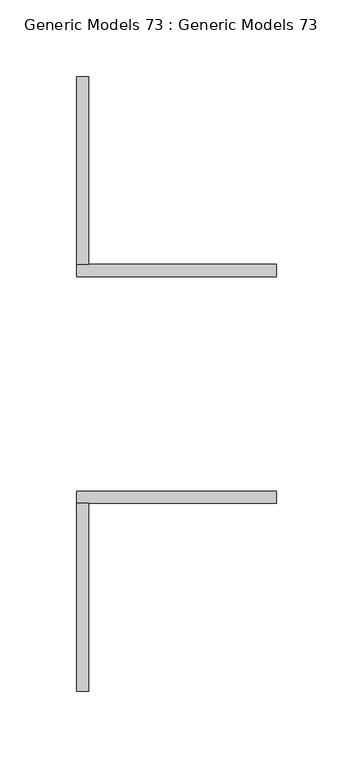
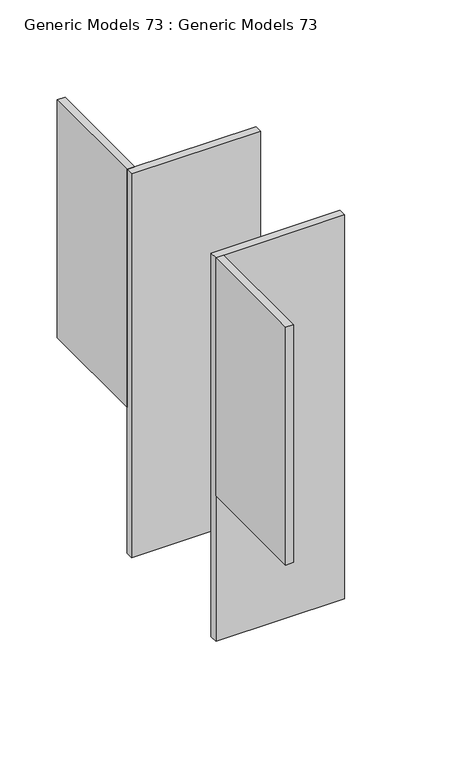
"""IFC4 building model written with IfcOpenShell, lengths in millimetres: proxy geometry, Generic Models 73 : Generic Models 73."""

import ifcopenshell
import ifcopenshell.guid

model = None  # the IFC model being written
_history = None  # IfcOwnerHistory: only IFC2X3 demands one
_inside = {}  # id of a spatial element -> (the spatial element, [elements in it])
_under = {}  # id of a project, library or spatial element -> (it, [spatial elements below it])
_declared = {}  # id of a project -> (the project, [libraries it declares])
_typed = {}  # id of a type object -> (the type object, [elements of that type])
_made_of = {}  # id of a material, layer set ... -> (it, [elements and type objects made of it])


def new_model(schema):
    """Start an empty IFC model of exactly this schema.

    Asked for "IFC4X3", IfcOpenShell would pick the latest addendum, in which some entities
    have other attributes; the version numbers below select the first issue.
    IFC2X3 requires an IfcOwnerHistory on every rooted entity: one is made here for all.
    """
    global model, _history
    if schema == "IFC4X3":
        model = ifcopenshell.file(schema_version=(4, 3, 0, 0))
    else:
        model = ifcopenshell.file(schema=schema)
    _inside.clear()
    _under.clear()
    _declared.clear()
    _typed.clear()
    _made_of.clear()
    _history = None
    if model.schema == "IFC2X3":
        org = make("IfcOrganization", Name="unknown")
        user = make(
            "IfcPersonAndOrganization",
            ThePerson=make("IfcPerson", FamilyName="unknown"),
            TheOrganization=org,
        )
        app = make(
            "IfcApplication",
            ApplicationDeveloper=org,
            Version="unknown",
            ApplicationFullName="unknown",
            ApplicationIdentifier="unknown",
        )
        _history = make(
            "IfcOwnerHistory",
            OwningUser=user,
            OwningApplication=app,
            ChangeAction="ADDED",
            CreationDate=0,
        )
    return model


def make(cls, **values):
    """One entity of the class cls with the attributes given. An attribute that is None is left unset."""
    return model.create_entity(
        cls, **{name: value for name, value in values.items() if value is not None}
    )


def rooted(cls, **values):
    """An entity with a GlobalId (a new one), such as an element, a storey or a relation."""
    return make(cls, GlobalId=ifcopenshell.guid.new(), OwnerHistory=_history, **values)


def si_unit(unit_type, name, prefix=None):
    """IfcSIUnit, for example si_unit("LENGTHUNIT", "METRE", prefix="MILLI")."""
    return make("IfcSIUnit", UnitType=unit_type, Prefix=prefix, Name=name)


def assignment(units):
    """IfcUnitAssignment: the units of a project."""
    return None if units is None else make("IfcUnitAssignment", Units=units)


def point(xyz):
    """IfcCartesianPoint."""
    return None if xyz is None else make("IfcCartesianPoint", Coordinates=xyz)


def direction(xyz):
    """IfcDirection."""
    return None if xyz is None else make("IfcDirection", DirectionRatios=xyz)


def frame(location, z_axis=None, x_axis=None):
    """IfcAxis2Placement3D, a coordinate frame: its origin and axes. An axis left out is left unset."""
    return make(
        "IfcAxis2Placement3D",
        Location=point(location),
        Axis=direction(z_axis),
        RefDirection=direction(x_axis),
    )


def origin():
    """The frame at (0, 0, 0) with its axes left unset."""
    return frame((0.0, 0.0, 0.0))


def place(relative_to, where):
    """IfcLocalPlacement: puts the frame where relative to a parent placement (None: the world)."""
    return make(
        "IfcLocalPlacement", PlacementRelTo=relative_to, RelativePlacement=where
    )


def context(
    kind, dimensions, precision=None, world=None, true_north=None, identifier=None
):
    """IfcGeometricRepresentationContext, for example the 3D "Model" context."""
    return make(
        "IfcGeometricRepresentationContext",
        ContextIdentifier=identifier,
        ContextType=kind,
        CoordinateSpaceDimension=dimensions,
        Precision=precision,
        WorldCoordinateSystem=world,
        TrueNorth=true_north,
    )


def project(units=None, contexts=None):
    """IfcProject with its units and contexts."""
    return rooted(
        "IfcProject",
        Name="project",
        RepresentationContexts=contexts,
        UnitsInContext=assignment(units),
    )


def spatial(cls, under=None, at=None, **own):
    """A site, building, storey or space (cls), placed at a placement, below another one or the project."""
    s = rooted(cls, ObjectPlacement=at, **own)
    if under is not None:
        _under.setdefault(under.id(), (under, []))[1].append(s)
    return s


def polyline(points):
    """IfcPolyline through the points."""
    return make("IfcPolyline", Points=[point(p) for p in points])


def outline(outer, holes=None, kind="AREA"):
    """IfcArbitraryClosedProfileDef: a profile drawn as a closed curve; with holes, ...WithVoids."""
    if holes is None:
        return make("IfcArbitraryClosedProfileDef", ProfileType=kind, OuterCurve=outer)
    return make(
        "IfcArbitraryProfileDefWithVoids",
        ProfileType=kind,
        OuterCurve=outer,
        InnerCurves=holes,
    )


def extrude(swept, where, along, depth):
    """IfcExtrudedAreaSolid: the profile swept, set in the frame where, extruded along a direction by depth."""
    return make(
        "IfcExtrudedAreaSolid",
        SweptArea=swept,
        Position=where,
        ExtrudedDirection=direction(along),
        Depth=depth,
    )


def shape(context_of_items, identifier, shape_type, items):
    """IfcShapeRepresentation: the items that make up one representation, for example the "Body"."""
    return make(
        "IfcShapeRepresentation",
        ContextOfItems=context_of_items,
        RepresentationIdentifier=identifier,
        RepresentationType=shape_type,
        Items=items,
    )


def source(mapping_origin, context_of_items, identifier, shape_type, items):
    """IfcRepresentationMap: a shape defined once, which mapped items show again and again."""
    return make(
        "IfcRepresentationMap",
        MappingOrigin=mapping_origin,
        MappedRepresentation=shape(context_of_items, identifier, shape_type, items),
    )


def transform(
    local_origin,
    x_axis=None,
    y_axis=None,
    z_axis=None,
    scale=None,
    scale2=None,
    scale3=None,
    uniform=True,
):
    """IfcCartesianTransformationOperator3D, or its non-uniform kind. x_axis, y_axis, z_axis: its Axis1, 2, 3."""
    if uniform:
        return make(
            "IfcCartesianTransformationOperator3D",
            Axis1=direction(x_axis),
            Axis2=direction(y_axis),
            LocalOrigin=point(local_origin),
            Scale=scale,
            Axis3=direction(z_axis),
        )
    return make(
        "IfcCartesianTransformationOperator3DnonUniform",
        Axis1=direction(x_axis),
        Axis2=direction(y_axis),
        LocalOrigin=point(local_origin),
        Scale=scale,
        Axis3=direction(z_axis),
        Scale2=scale2,
        Scale3=scale3,
    )


def mapped(mapping_source, mapping_target):
    """IfcMappedItem: shows the shape of a source again, moved by a transform."""
    return make(
        "IfcMappedItem", MappingSource=mapping_source, MappingTarget=mapping_target
    )


def made_of(thing, what):
    """Note that an element or type object is made of a material, layer set ...; save() writes the relation."""
    if what is not None:
        _made_of.setdefault(what.id(), (what, []))[1].append(thing)
    return thing


def element(
    cls,
    number,
    at=None,
    inside=None,
    cuts=None,
    type_object=None,
    material=None,
    context=None,
    identifier="Body",
    shape_type=None,
    held_by="IfcProductDefinitionShape",
    body=None,
    shapes=None,
    **own,
):
    """One element of the class cls, such as IfcWall. Its Tag is "e" and its number.

    at: its placement. inside: the storey or other place that contains it. cuts: it is an
    opening in that element (IfcRelVoidsElement). A single representation is given by context,
    identifier, shape_type and body (its items); several are given by shapes. held_by: the class
    of the entity that holds the representations. save() writes the other relations.
    """
    e = rooted(cls, Tag="e%d" % number, ObjectPlacement=at, **own)
    if body is not None:
        shapes = [shape(context, identifier, shape_type, body)]
    if shapes is not None:
        e.Representation = make(held_by, Representations=shapes)
    if inside is not None:
        _inside.setdefault(inside.id(), (inside, []))[1].append(e)
    if cuts is not None:
        rooted(
            "IfcRelVoidsElement", RelatingBuildingElement=cuts, RelatedOpeningElement=e
        )
    if type_object is not None:
        _typed.setdefault(type_object.id(), (type_object, []))[1].append(e)
    return made_of(e, material)


def aggregate(whole, parts):
    """IfcRelAggregates: a whole, such as a stair, and the parts it consists of."""
    return rooted("IfcRelAggregates", RelatingObject=whole, RelatedObjects=parts)


def save(model, path):
    """Write the relations noted so far, then the file.

    IfcRelAggregates (storeys below a building ...), IfcRelContainedInSpatialStructure (elements
    in a storey), IfcRelDefinesByType, IfcRelAssociatesMaterial and IfcRelDeclares: one each for
    every whole, place, type object, material and project.
    """
    for whole, parts in _under.values():
        aggregate(whole, parts)
    for where, things in _inside.values():
        rooted(
            "IfcRelContainedInSpatialStructure",
            RelatedElements=things,
            RelatingStructure=where,
        )
    for kind, things in _typed.values():
        rooted("IfcRelDefinesByType", RelatedObjects=things, RelatingType=kind)
    for what, things in _made_of.values():
        rooted("IfcRelAssociatesMaterial", RelatedObjects=things, RelatingMaterial=what)
    for by, libraries in _declared.values():
        rooted("IfcRelDeclares", RelatingContext=by, RelatedDefinitions=libraries)
    model.write(path)


def generic_models_73_generic_models_73_c8f64cd2(model_context):
    return source(origin(), model_context, "Body", "SweptSolid", [
        extrude(outline(polyline([(31918.2596032, 36207.3957942), (31910.3221032, 36207.3957942), (31910.3221032, 36329.6332942), (31918.2596032, 36329.6332942), (31918.2596032, 36207.3957942)])), frame((0.0, 0.0, 271626.0125), z_axis=(0.0, 0.0, 1.0), x_axis=(1.0, 0.0, 0.0)), (0.0, 0.0, 1.0), 254.0),
        extrude(outline(polyline([(31910.3221032, 36607.4457942), (31918.2596032, 36607.4457942), (31918.2596032, 36485.2082942), (31910.3221032, 36485.2082942), (31910.3221032, 36607.4457942)])), frame((0.0, 0.0, 271626.0125), z_axis=(0.0, 0.0, 1.0), x_axis=(1.0, 0.0, 0.0)), (0.0, 0.0, 1.0), 254.0),
        extrude(outline(polyline([(32040.4971032, 36485.2082942), (32040.4971032, 36477.2707942), (31910.3221032, 36477.2707942), (31910.3221032, 36485.2082942), (32040.4971032, 36485.2082942)])), frame((0.0, 0.0, 271470.4375), z_axis=(0.0, 0.0, 1.0), x_axis=(1.0, 0.0, 0.0)), (0.0, 0.0, 1.0), 409.575),
        extrude(outline(polyline([(32040.4971032, 36337.5707942), (32040.4971032, 36329.6332942), (31910.3221032, 36329.6332942), (31910.3221032, 36337.5707942), (32040.4971032, 36337.5707942)])), frame((0.0, 0.0, 271470.4375), z_axis=(0.0, 0.0, 1.0), x_axis=(1.0, 0.0, 0.0)), (0.0, 0.0, 1.0), 409.575),
    ])


if __name__ == "__main__":
    model = new_model("IFC4")
    model_context = context("Model", 3, world=origin())
    ifc_project = project(units=[si_unit("LENGTHUNIT", "METRE", prefix="MILLI")], contexts=[model_context])
    site = spatial("IfcSite", under=ifc_project)
    building = spatial("IfcBuilding", under=site)
    placement = place(None, origin())
    generic_models_73_generic_models_73_shape = generic_models_73_generic_models_73_c8f64cd2(model_context)
    element("IfcBuildingElementProxy", 1, Name="Generic Models 73 : Generic Models 73", ObjectType="Generic Models 73 : Generic Models 73", at=placement, inside=building, context=model_context, shape_type="MappedRepresentation", body=[
        mapped(generic_models_73_generic_models_73_shape, transform((0.0, 0.0, 0.0), x_axis=(1.0, 0.0, 0.0), y_axis=(0.0, 1.0, 0.0), z_axis=(0.0, 0.0, 1.0))),
    ])
    save(model, "model.ifc")

# Revit data of these elements
# Element 1 (IfcBuildingElementProxy, "Generic Models 73 : Generic Models 73")
#   Materials on its faces: "5 1/8 x 10 x 0 5/16\" PLATE W/ 3 1\"DIA. THRU BOLTS", "5/16 x 9 x 0'-11\" SIDE PLATES  CAP\nW/ 2 3/4\"DIA. THRU BOLTS"
# Materials
#   "5 1/8 x 10 x 0 5/16\" PLATE W/ 3 1\"DIA. THRU BOLTS": class "Metal", colour RGB 199 199 199, transparency 0, Description = "Carbon steel", Cost = 0
#   "5/16 x 9 x 0'-11\" SIDE PLATES  CAP\nW/ 2 3/4\"DIA. THRU BOLTS": class "Metal", colour RGB 199 199 199, transparency 0, Description = "Carbon steel", Cost = 0
